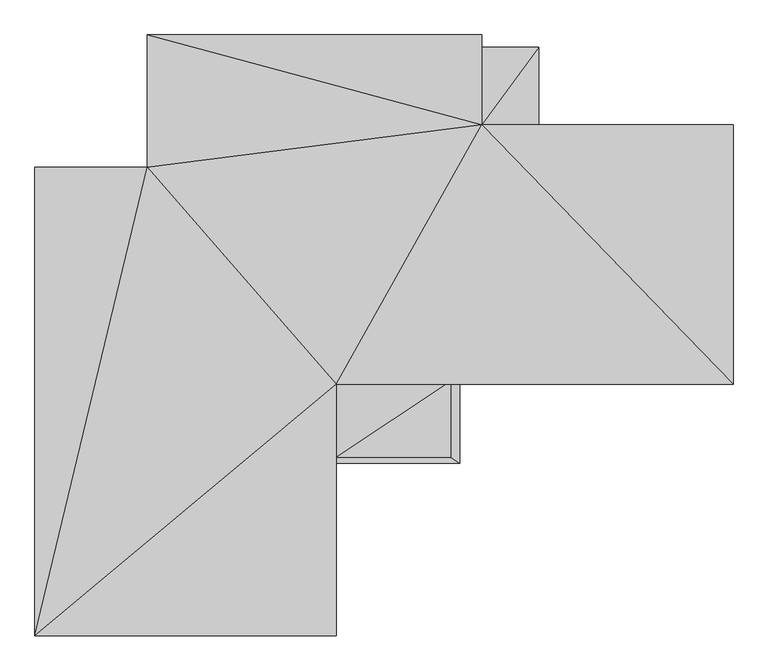
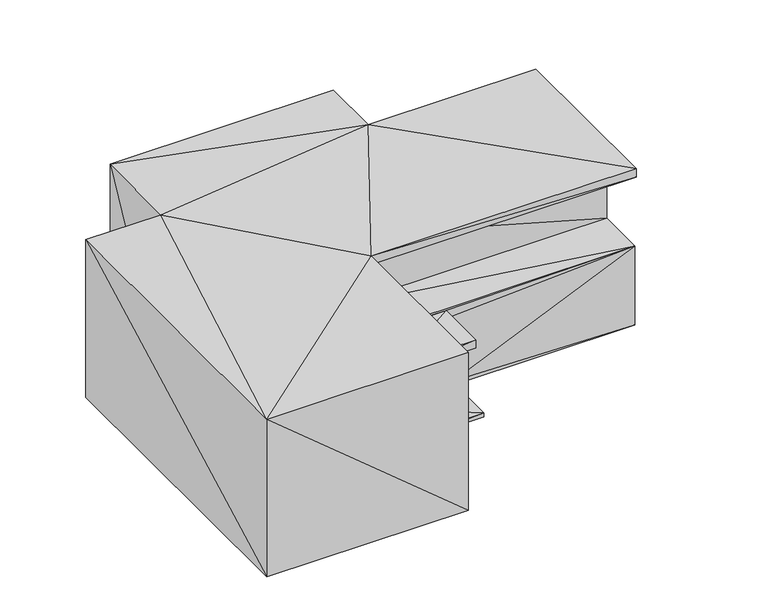
"""IFC4 building model written with IfcOpenShell, lengths in millimetres: geographic element geometry, Enscape AssetDefinition - Surrounding Building 017 Family House : Enscape AssetDefinition - Surrounding Building 017 Family House."""

from ifc_helpers import new_model, si_unit, origin, place, context, project, spatial, faceted_brep, source, transform, mapped, element, save


def geographic_element_ab947704(model_context):
    return source(origin(), model_context, "Body", "Brep", [
        faceted_brep([(18.8970007, 1401.2249708, 153.3440053), (18.8970007, 1401.2249708, 0.0), (2983.3929539, 1401.2249708, 153.3440053), (-4151.4849663, 8536.4017487, 0.0), (-1721.3959694, 8536.4017487, 0.0), (2983.3929539, 1401.2249708, 0.0), (18.8970007, -2755.7048798, 0.0), (2983.3929539, 3381.6308975, 0.0), (-7244.5340157, -2755.7048798, 0.0), (-4536.4360809, 8536.4017487, 0.0), (2983.3929539, 3381.6308975, 153.3440053), (9570.7101822, 3381.6308975, 0.0), (3133.5070133, 9554.9755096, 0.0), (3518.4578896, 9554.9755096, 0.0), (18.8970007, 3381.6308975, 153.3440053), (9570.7101822, 3381.6308975, 3005.2630901), (2773.4398842, 3381.6308975, 2625.7069111), (18.8970007, 3381.6308975, 2625.7069111), (18.8970007, 1542.9199934, 2625.7069111), (2773.4398842, 3381.6308975, 2923.915863), (2773.4398842, 1542.9199934, 2625.7069111), (2773.4398842, 1542.9199934, 2923.915863), (18.8970007, 1542.9199934, 2923.915863), (18.8970007, 3381.6308975, 2923.915863), (18.8970007, 3381.6308975, 3005.2630901), (18.8970007, -2755.7048798, 6010.0002289), (18.8979991, 3304.9330711, 5686.8710518), (-7244.5340157, -2755.7048798, 6010.0002289), (18.8979991, 3304.9330711, 6010.0002289), (9570.7101822, 3304.9340248, 5686.8710518), (9570.7101822, 5143.4860229, 5686.8710518), (18.8979991, 5143.4860229, 5686.8710518), (-4536.4360809, 8536.4017487, 6010.0002289), (9570.7101822, 3304.9340248, 6010.0002289), (3518.4578896, 9554.9755096, 6010.0002289), (9570.7101822, 5143.4860229, 3005.2630901), (9570.7101822, 9554.977417, 6010.0002289), (18.8970007, 5143.4860229, 3005.2630901), (9570.7101822, 9554.977417, 0.0), (4888.5769844, 9554.9755096, 2942.7149296), (4888.5779381, 9554.9755096, 2596.6930389), (3518.4578896, 9554.9755096, 2596.6911316), (3518.4578896, 11421.3209152, 2596.6911316), (3518.4569359, 11718.6288834, 0.001), (4888.5779381, 11421.3209152, 2596.6930389), (4888.5769844, 11421.3209152, 2942.7149296), (3518.4569359, 11421.3209152, 2942.7139759), (3518.4578896, 9554.977417, 2942.7139759), (3518.4569359, 11718.6288834, 6010.0011826), (-4536.4370346, 11718.6279297, 6010.0002289), (-4151.48592, 11718.6279297, 2620.4738617), (3133.5070133, 11718.6288834, 2620.4750538), (-4536.4370346, 11718.6279297, 0.0), (-7244.5340157, 8536.4017487, 0.0), (-7244.5340157, 8536.4017487, 6010.0002289), (-4151.4849663, 11718.6279297, 0.0), (-4151.4849663, 8536.4017487, 2619.5931435), (-1721.3969231, 8536.4017487, 2619.5940971), (-1721.3959694, 9554.9755096, 2619.8749542), (-1721.3959694, 9554.9755096, 0.0), (3133.5070133, 9554.977417, 2619.8759079), (3133.5070133, 11718.6288834, 0.0)], [[[0, 1, 2]], [[1, 3, 4]], [[2, 1, 5]], [[0, 6, 1]], [[1, 7, 5]], [[8, 1, 6]], [[9, 1, 8]], [[4, 7, 1]], [[1, 9, 3]], [[7, 10, 5]], [[5, 10, 2]], [[10, 7, 11]], [[7, 4, 12]], [[7, 12, 13]], [[7, 13, 11]], [[10, 14, 2]], [[15, 16, 10]], [[10, 11, 15]], [[16, 14, 10]], [[2, 14, 0]], [[16, 17, 14]], [[18, 0, 14]], [[18, 14, 17]], [[16, 19, 20]], [[20, 17, 16]], [[16, 15, 19]], [[18, 17, 20]], [[20, 21, 18]], [[22, 6, 18]], [[18, 21, 22]], [[18, 6, 0]], [[20, 19, 21]], [[21, 19, 22]], [[22, 19, 23]], [[19, 15, 24]], [[19, 24, 23]], [[22, 25, 6]], [[22, 26, 25]], [[22, 23, 24]], [[22, 24, 26]], [[8, 6, 27]], [[27, 6, 25]], [[28, 27, 25]], [[26, 28, 25]], [[26, 29, 28]], [[29, 26, 30]], [[26, 24, 31]], [[30, 26, 31]], [[28, 32, 27]], [[28, 29, 33]], [[34, 28, 33]], [[28, 34, 32]], [[30, 33, 29]], [[35, 36, 30]], [[30, 31, 35]], [[30, 36, 33]], [[35, 31, 37]], [[31, 24, 37]], [[35, 37, 15]], [[35, 11, 38]], [[35, 38, 36]], [[11, 35, 15]], [[15, 37, 24]], [[11, 13, 38]], [[39, 36, 38]], [[40, 38, 13]], [[39, 38, 40]], [[40, 13, 41]], [[42, 41, 13]], [[42, 13, 43]], [[13, 12, 43]], [[40, 41, 44]], [[39, 40, 45]], [[45, 40, 44]], [[44, 41, 42]], [[43, 46, 42]], [[42, 46, 44]], [[44, 46, 45]], [[46, 47, 45]], [[45, 47, 39]], [[46, 48, 34]], [[46, 34, 47]], [[43, 48, 46]], [[34, 39, 47]], [[36, 39, 34]], [[34, 33, 36]], [[49, 34, 48]], [[32, 34, 49]], [[49, 48, 50]], [[51, 48, 43]], [[50, 48, 51]], [[52, 9, 49]], [[50, 52, 49]], [[49, 9, 32]], [[9, 53, 32]], [[32, 53, 54]], [[27, 32, 54]], [[9, 8, 53]], [[55, 9, 52]], [[3, 9, 55]], [[50, 55, 52]], [[3, 55, 56]], [[56, 55, 50]], [[56, 4, 3]], [[57, 4, 56]], [[58, 57, 56]], [[58, 56, 50]], [[4, 57, 59]], [[12, 4, 59]], [[59, 57, 58]], [[58, 51, 60]], [[58, 60, 59]], [[58, 50, 51]], [[59, 60, 12]], [[12, 60, 61]], [[43, 12, 61]], [[61, 60, 51]], [[51, 43, 61]], [[53, 8, 54]], [[54, 8, 27]]]),
    ])


if __name__ == "__main__":
    model = new_model("IFC4")
    model_context = context("Model", 3, world=origin())
    ifc_project = project(units=[si_unit("LENGTHUNIT", "METRE", prefix="MILLI")], contexts=[model_context])
    site = spatial("IfcSite", under=ifc_project)
    building = spatial("IfcBuilding", under=site)
    placement = place(None, origin())
    geographic_element_shape = geographic_element_ab947704(model_context)
    element("IfcGeographicElement", 1, ObjectType="Enscape AssetDefinition - Surrounding Building 017 Family House : Enscape AssetDefinition - Surrounding Building 017 Family House", at=placement, inside=building, context=model_context, shape_type="MappedRepresentation", body=[
        mapped(geographic_element_shape, transform((0.0, 0.0, 0.0), x_axis=(1.0, 0.0, 0.0), y_axis=(0.0, 1.0, 0.0), z_axis=(0.0, 0.0, 1.0))),
    ])
    save(model, "model.ifc")

# Revit data of these elements
# Type "Enscape AssetDefinition - Surrounding Building 017 Family House : Enscape AssetDefinition - Surrounding Building 017 Family House"
#   EnscapeAssetSource = "REMOTE"
#   EnscapeAssetId = "2a87e29e-e425-4825-bf71-8528d1ebcdce"
#   Height = 6010.001 mm
#   EnscapeNativeAssetHeight = 6010.001 mm
#   Default Elevation = 0
